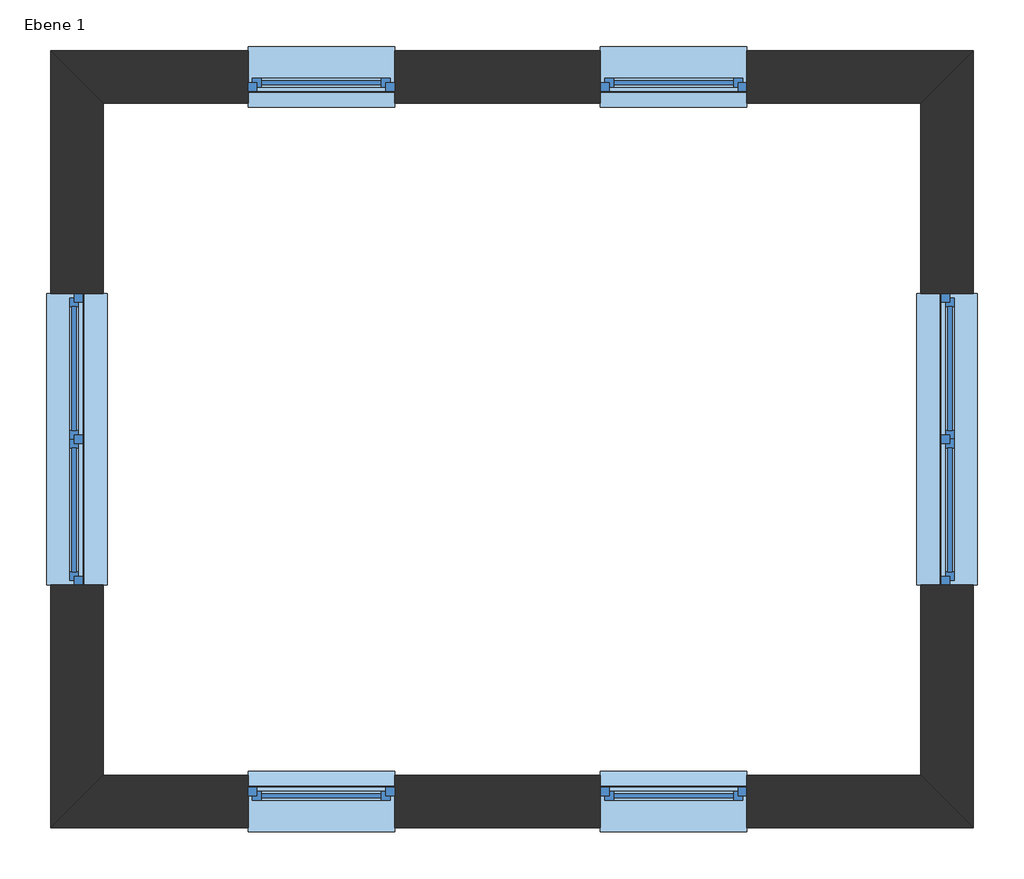
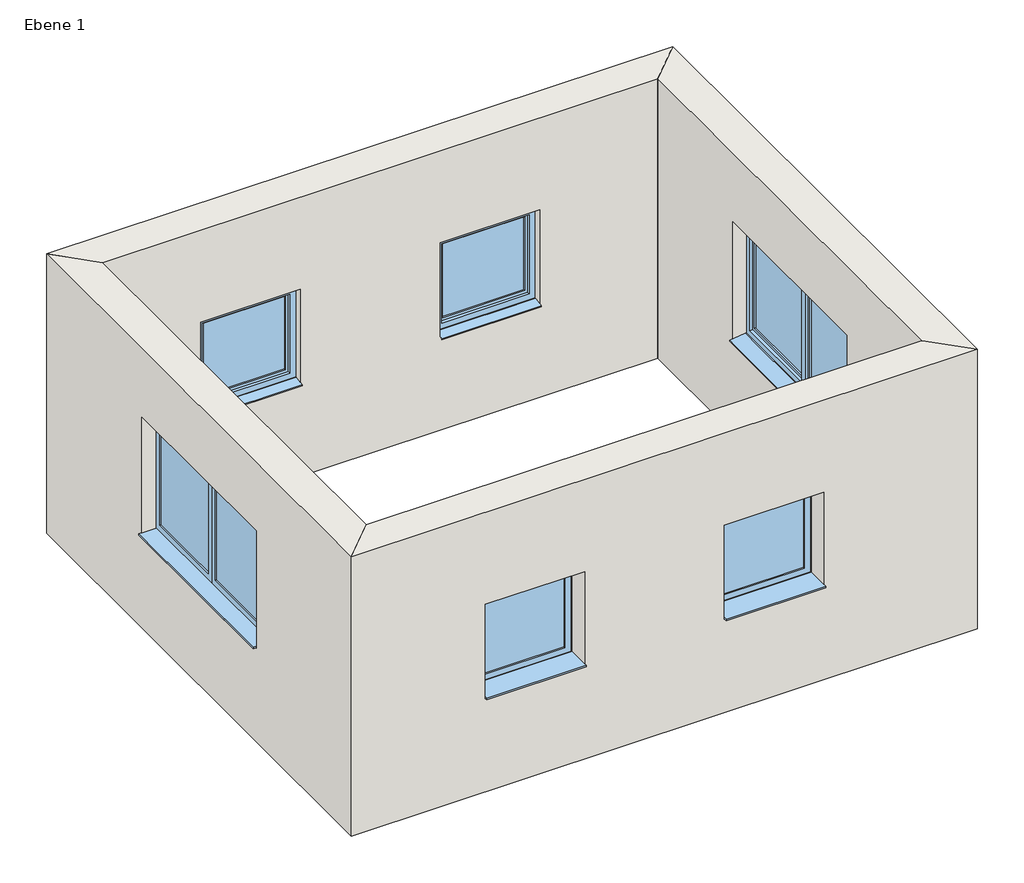
# One storey: 6 windows, 4 walls.
"""IFC4 building model written with IfcOpenShell, lengths in millimetres."""

import ifcopenshell
import ifcopenshell.guid

model = None  # the IFC model being written
_history = None  # IfcOwnerHistory: only IFC2X3 demands one
_inside = {}  # id of a spatial element -> (the spatial element, [elements in it])
_under = {}  # id of a project, library or spatial element -> (it, [spatial elements below it])
_declared = {}  # id of a project -> (the project, [libraries it declares])
_typed = {}  # id of a type object -> (the type object, [elements of that type])
_made_of = {}  # id of a material, layer set ... -> (it, [elements and type objects made of it])


def new_model(schema):
    """Start an empty IFC model of exactly this schema.

    Asked for "IFC4X3", IfcOpenShell would pick the latest addendum, in which some entities
    have other attributes; the version numbers below select the first issue.
    IFC2X3 requires an IfcOwnerHistory on every rooted entity: one is made here for all.
    """
    global model, _history
    if schema == "IFC4X3":
        model = ifcopenshell.file(schema_version=(4, 3, 0, 0))
    else:
        model = ifcopenshell.file(schema=schema)
    _inside.clear()
    _under.clear()
    _declared.clear()
    _typed.clear()
    _made_of.clear()
    _history = None
    if model.schema == "IFC2X3":
        org = make("IfcOrganization", Name="unknown")
        user = make(
            "IfcPersonAndOrganization",
            ThePerson=make("IfcPerson", FamilyName="unknown"),
            TheOrganization=org,
        )
        app = make(
            "IfcApplication",
            ApplicationDeveloper=org,
            Version="unknown",
            ApplicationFullName="unknown",
            ApplicationIdentifier="unknown",
        )
        _history = make(
            "IfcOwnerHistory",
            OwningUser=user,
            OwningApplication=app,
            ChangeAction="ADDED",
            CreationDate=0,
        )
    return model


def make(cls, **values):
    """One entity of the class cls with the attributes given. An attribute that is None is left unset."""
    return model.create_entity(
        cls, **{name: value for name, value in values.items() if value is not None}
    )


def rooted(cls, **values):
    """An entity with a GlobalId (a new one), such as an element, a storey or a relation."""
    return make(cls, GlobalId=ifcopenshell.guid.new(), OwnerHistory=_history, **values)


def si_unit(unit_type, name, prefix=None):
    """IfcSIUnit, for example si_unit("LENGTHUNIT", "METRE", prefix="MILLI")."""
    return make("IfcSIUnit", UnitType=unit_type, Prefix=prefix, Name=name)


def assignment(units):
    """IfcUnitAssignment: the units of a project."""
    return None if units is None else make("IfcUnitAssignment", Units=units)


def point(xyz):
    """IfcCartesianPoint."""
    return None if xyz is None else make("IfcCartesianPoint", Coordinates=xyz)


def direction(xyz):
    """IfcDirection."""
    return None if xyz is None else make("IfcDirection", DirectionRatios=xyz)


def frame(location, z_axis=None, x_axis=None):
    """IfcAxis2Placement3D, a coordinate frame: its origin and axes. An axis left out is left unset."""
    return make(
        "IfcAxis2Placement3D",
        Location=point(location),
        Axis=direction(z_axis),
        RefDirection=direction(x_axis),
    )


def origin():
    """The frame at (0, 0, 0) with its axes left unset."""
    return frame((0.0, 0.0, 0.0))


def place(relative_to, where):
    """IfcLocalPlacement: puts the frame where relative to a parent placement (None: the world)."""
    return make(
        "IfcLocalPlacement", PlacementRelTo=relative_to, RelativePlacement=where
    )


def context(
    kind, dimensions, precision=None, world=None, true_north=None, identifier=None
):
    """IfcGeometricRepresentationContext, for example the 3D "Model" context."""
    return make(
        "IfcGeometricRepresentationContext",
        ContextIdentifier=identifier,
        ContextType=kind,
        CoordinateSpaceDimension=dimensions,
        Precision=precision,
        WorldCoordinateSystem=world,
        TrueNorth=true_north,
    )


def project(units=None, contexts=None):
    """IfcProject with its units and contexts."""
    return rooted(
        "IfcProject",
        Name="project",
        RepresentationContexts=contexts,
        UnitsInContext=assignment(units),
    )


def spatial(cls, under=None, at=None, **own):
    """A site, building, storey or space (cls), placed at a placement, below another one or the project."""
    s = rooted(cls, ObjectPlacement=at, **own)
    if under is not None:
        _under.setdefault(under.id(), (under, []))[1].append(s)
    return s


def polyline(points):
    """IfcPolyline through the points."""
    return make("IfcPolyline", Points=[point(p) for p in points])


def outline(outer, holes=None, kind="AREA"):
    """IfcArbitraryClosedProfileDef: a profile drawn as a closed curve; with holes, ...WithVoids."""
    if holes is None:
        return make("IfcArbitraryClosedProfileDef", ProfileType=kind, OuterCurve=outer)
    return make(
        "IfcArbitraryProfileDefWithVoids",
        ProfileType=kind,
        OuterCurve=outer,
        InnerCurves=holes,
    )


def extrude(swept, where, along, depth):
    """IfcExtrudedAreaSolid: the profile swept, set in the frame where, extruded along a direction by depth."""
    return make(
        "IfcExtrudedAreaSolid",
        SweptArea=swept,
        Position=where,
        ExtrudedDirection=direction(along),
        Depth=depth,
    )


def faces_of(points, faces, orient=None, outer=None):
    """IfcFace entities. A face is a list of loops; a loop is a list of indices into points, from 0.

    orient and outer hold one flag for each loop. By default every Orientation is true, the
    first loop of a face is its IfcFaceOuterBound and the others are IfcFaceBound.
    """
    made = []
    for i, loops in enumerate(faces):
        bounds = []
        for j, loop in enumerate(loops):
            is_outer = j == 0 if outer is None else outer[i][j]
            bounds.append(
                make(
                    "IfcFaceOuterBound" if is_outer else "IfcFaceBound",
                    Bound=make("IfcPolyLoop", Polygon=[points[k] for k in loop]),
                    Orientation=True if orient is None else orient[i][j],
                )
            )
        made.append(make("IfcFace", Bounds=bounds))
    return made


def faceted_brep(points, faces, orient=None, outer=None, voids=None):
    """IfcFacetedBrep: a solid bounded by flat faces; with voids (closed shells), ...WithVoids."""
    shared = [point(p) for p in points]
    hull = make("IfcClosedShell", CfsFaces=faces_of(shared, faces, orient, outer))
    if voids is None:
        return make("IfcFacetedBrep", Outer=hull)
    return make(
        "IfcFacetedBrepWithVoids",
        Outer=hull,
        Voids=[
            make(cls, CfsFaces=faces_of(shared, fs, o, b)) for cls, fs, o, b in voids
        ],
    )


def shape(context_of_items, identifier, shape_type, items):
    """IfcShapeRepresentation: the items that make up one representation, for example the "Body"."""
    return make(
        "IfcShapeRepresentation",
        ContextOfItems=context_of_items,
        RepresentationIdentifier=identifier,
        RepresentationType=shape_type,
        Items=items,
    )


def source(mapping_origin, context_of_items, identifier, shape_type, items):
    """IfcRepresentationMap: a shape defined once, which mapped items show again and again."""
    return make(
        "IfcRepresentationMap",
        MappingOrigin=mapping_origin,
        MappedRepresentation=shape(context_of_items, identifier, shape_type, items),
    )


def transform(
    local_origin,
    x_axis=None,
    y_axis=None,
    z_axis=None,
    scale=None,
    scale2=None,
    scale3=None,
    uniform=True,
):
    """IfcCartesianTransformationOperator3D, or its non-uniform kind. x_axis, y_axis, z_axis: its Axis1, 2, 3."""
    if uniform:
        return make(
            "IfcCartesianTransformationOperator3D",
            Axis1=direction(x_axis),
            Axis2=direction(y_axis),
            LocalOrigin=point(local_origin),
            Scale=scale,
            Axis3=direction(z_axis),
        )
    return make(
        "IfcCartesianTransformationOperator3DnonUniform",
        Axis1=direction(x_axis),
        Axis2=direction(y_axis),
        LocalOrigin=point(local_origin),
        Scale=scale,
        Axis3=direction(z_axis),
        Scale2=scale2,
        Scale3=scale3,
    )


def mapped(mapping_source, mapping_target):
    """IfcMappedItem: shows the shape of a source again, moved by a transform."""
    return make(
        "IfcMappedItem", MappingSource=mapping_source, MappingTarget=mapping_target
    )


def made_of(thing, what):
    """Note that an element or type object is made of a material, layer set ...; save() writes the relation."""
    if what is not None:
        _made_of.setdefault(what.id(), (what, []))[1].append(thing)
    return thing


def element(
    cls,
    number,
    at=None,
    inside=None,
    cuts=None,
    type_object=None,
    material=None,
    context=None,
    identifier="Body",
    shape_type=None,
    held_by="IfcProductDefinitionShape",
    body=None,
    shapes=None,
    **own,
):
    """One element of the class cls, such as IfcWall. Its Tag is "e" and its number.

    at: its placement. inside: the storey or other place that contains it. cuts: it is an
    opening in that element (IfcRelVoidsElement). A single representation is given by context,
    identifier, shape_type and body (its items); several are given by shapes. held_by: the class
    of the entity that holds the representations. save() writes the other relations.
    """
    e = rooted(cls, Tag="e%d" % number, ObjectPlacement=at, **own)
    if body is not None:
        shapes = [shape(context, identifier, shape_type, body)]
    if shapes is not None:
        e.Representation = make(held_by, Representations=shapes)
    if inside is not None:
        _inside.setdefault(inside.id(), (inside, []))[1].append(e)
    if cuts is not None:
        rooted(
            "IfcRelVoidsElement", RelatingBuildingElement=cuts, RelatedOpeningElement=e
        )
    if type_object is not None:
        _typed.setdefault(type_object.id(), (type_object, []))[1].append(e)
    return made_of(e, material)


def aggregate(whole, parts):
    """IfcRelAggregates: a whole, such as a stair, and the parts it consists of."""
    return rooted("IfcRelAggregates", RelatingObject=whole, RelatedObjects=parts)


def save(model, path):
    """Write the relations noted so far, then the file.

    IfcRelAggregates (storeys below a building ...), IfcRelContainedInSpatialStructure (elements
    in a storey), IfcRelDefinesByType, IfcRelAssociatesMaterial and IfcRelDeclares: one each for
    every whole, place, type object, material and project.
    """
    for whole, parts in _under.values():
        aggregate(whole, parts)
    for where, things in _inside.values():
        rooted(
            "IfcRelContainedInSpatialStructure",
            RelatedElements=things,
            RelatingStructure=where,
        )
    for kind, things in _typed.values():
        rooted("IfcRelDefinesByType", RelatedObjects=things, RelatingType=kind)
    for what, things in _made_of.values():
        rooted("IfcRelAssociatesMaterial", RelatedObjects=things, RelatingMaterial=what)
    for by, libraries in _declared.values():
        rooted("IfcRelDeclares", RelatingContext=by, RelatedDefinitions=libraries)
    model.write(path)


def fenster_1_flg_variabel_fenster_1_flg_variabel_3_8a378bad(model_context):
    return source(origin(), model_context, "Body", "SolidModel", [
        extrude(outline(polyline([(2010.0, 505.0), (2010.0, -505.0), (1000.0, -505.0), (1000.0, 505.0), (2010.0, 505.0)]), holes=[polyline([(1930.0, 445.0), (1080.0, 445.0), (1080.0, -445.0), (1930.0, -445.0), (1930.0, 445.0)])]), frame((0.0, 40.0, 0.0), z_axis=(0.0, 1.0, 0.0), x_axis=(0.0, 0.0, 1.0)), (0.0, 0.0, 1.0), 60.0),
        faceted_brep([(475.0, 40.0, 1960.0), (475.0, 10.0, 1960.0), (475.0, 10.0, 1050.0), (475.0, 40.0, 1050.0), (-475.0, 10.0, 1960.0), (-475.0, 10.0, 1050.0), (415.0, 10.0, 1110.0), (-415.0, 10.0, 1110.0), (-415.0, 10.0, 1900.0), (415.0, 10.0, 1900.0), (-475.0, 40.0, 1050.0), (-475.0, 40.0, 1960.0), (445.0, 40.0, 1930.0), (-445.0, 40.0, 1930.0), (-445.0, 40.0, 1080.0), (445.0, 40.0, 1080.0), (445.0, 70.0, 1930.0), (445.0, 70.0, 1080.0), (-445.0, 70.0, 1080.0), (-445.0, 70.0, 1930.0), (415.0, 70.0, 1900.0), (-415.0, 70.0, 1900.0), (-415.0, 70.0, 1110.0), (415.0, 70.0, 1110.0)], [[[0, 1, 2, 3]], [[1, 4, 5, 2], [6, 7, 8, 9]], [[3, 2, 5, 10]], [[3, 10, 11, 0], [12, 13, 14, 15]], [[16, 12, 15, 17]], [[17, 15, 14, 18]], [[17, 18, 19, 16], [20, 21, 22, 23]], [[9, 20, 23, 6]], [[6, 23, 22, 7]], [[10, 5, 4, 11]], [[18, 14, 13, 19]], [[7, 22, 21, 8]], [[11, 4, 1, 0]], [[19, 13, 12, 16]], [[8, 21, 20, 9]]]),
        extrude(outline(polyline([(-505.0, -210.0), (-505.0, 40.0), (505.0, 40.0), (505.0, -210.0), (-505.0, -210.0)])), frame((0.0, 0.0, 1005.0), z_axis=(0.0, 0.0, 1.0), x_axis=(1.0, 0.0, 0.0)), (0.0, 0.0, 1.0), 15.0),
        extrude(outline(polyline([(110.0221543, 1020.0), (210.0, 1000.0), (210.0, 990.0), (208.0, 990.0), (208.0, 998.3604634), (109.8240723, 1018.0), (100.0, 1018.0), (100.0, 1020.0), (110.0221543, 1020.0)])), frame((-505.0, 0.0, 0.0), z_axis=(1.0, 0.0, 0.0), x_axis=(0.0, 1.0, 0.0)), (0.0, 0.0, 1.0), 1010.0),
        extrude(outline(polyline([(415.0, 25.0), (-415.0, 25.0), (-415.0, 55.0), (415.0, 55.0), (415.0, 25.0)])), frame((0.0, 0.0, 1110.0), z_axis=(0.0, 0.0, 1.0), x_axis=(1.0, 0.0, 0.0)), (0.0, 0.0, 1.0), 790.0),
    ])


def fenster_2_flg_variabel_fenster_2_flg_variabel_3_03287464(model_context):
    return source(origin(), model_context, "Body", "SolidModel", [
        extrude(outline(polyline([(60.0, -5.0), (915.0, -5.0), (915.0, -35.0), (60.0, -35.0), (60.0, -5.0)])), frame((0.0, 0.0, 1110.0), z_axis=(0.0, 0.0, 1.0), x_axis=(1.0, 0.0, 0.0)), (0.0, 0.0, 1.0), 1040.0),
        extrude(outline(polyline([(-915.0, -5.0), (-60.0, -5.0), (-60.0, -35.0), (-915.0, -35.0), (-915.0, -5.0)])), frame((0.0, 0.0, 1110.0), z_axis=(0.0, 0.0, 1.0), x_axis=(1.0, 0.0, 0.0)), (0.0, 0.0, 1.0), 1040.0),
        extrude(outline(polyline([(-1005.0, -210.0), (-1005.0, -20.0), (1005.0, -20.0), (1005.0, -210.0), (-1005.0, -210.0)])), frame((0.0, 0.0, 1005.0), z_axis=(0.0, 0.0, 1.0), x_axis=(1.0, 0.0, 0.0)), (0.0, 0.0, 1.0), 15.0),
        extrude(outline(polyline([(50.0221543, 1020.0), (210.0, 1000.0), (210.0, 990.0), (208.0, 990.0), (208.0, 998.3604634), (49.8240723, 1018.0), (40.0, 1018.0), (40.0, 1020.0), (50.0221543, 1020.0)])), frame((-1005.0, 0.0, 0.0), z_axis=(1.0, 0.0, 0.0), x_axis=(0.0, 1.0, 0.0)), (0.0, 0.0, 1.0), 2010.0),
        extrude(outline(polyline([(30.0, -20.0), (-30.0, -20.0), (-30.0, 40.0), (30.0, 40.0), (30.0, -20.0)])), frame((0.0, 0.0, 1080.0), z_axis=(0.0, 0.0, 1.0), x_axis=(1.0, 0.0, 0.0)), (0.0, 0.0, 1.0), 1100.0),
        extrude(outline(polyline([(2260.0, -1005.0), (1000.0, -1005.0), (1000.0, 1005.0), (2260.0, 1005.0), (2260.0, -1005.0)]), holes=[polyline([(2180.0, -945.0), (2180.0, 945.0), (1080.0, 945.0), (1080.0, -945.0), (2180.0, -945.0)])]), frame((0.0, -20.0, 0.0), z_axis=(0.0, 1.0, 0.0), x_axis=(0.0, 0.0, 1.0)), (0.0, 0.0, 1.0), 60.0),
        faceted_brep([(-945.0, -20.0, 1080.0), (-945.0, 10.0, 1080.0), (-30.0, 10.0, 1080.0), (-30.0, -20.0, 1080.0), (-30.0, 10.0, 2180.0), (-30.0, -20.0, 2180.0), (-945.0, 10.0, 2180.0), (-60.0, 10.0, 2150.0), (-915.0, 10.0, 2150.0), (-915.0, 10.0, 1110.0), (-60.0, 10.0, 1110.0), (0.0, -20.0, 1050.0), (-975.0, -20.0, 1050.0), (-975.0, -20.0, 2210.0), (0.0, -20.0, 2210.0), (-945.0, -20.0, 2180.0), (-975.0, -50.0, 1050.0), (0.0, -50.0, 1050.0), (0.0, -50.0, 2210.0), (-975.0, -50.0, 2210.0), (-60.0, -50.0, 1110.0), (-915.0, -50.0, 1110.0), (-915.0, -50.0, 2150.0), (-60.0, -50.0, 2150.0)], [[[0, 1, 2, 3]], [[3, 2, 4, 5]], [[2, 1, 6, 4], [7, 8, 9, 10]], [[11, 12, 13, 14], [5, 15, 0, 3]], [[16, 12, 11, 17]], [[17, 11, 14, 18]], [[18, 19, 16, 17], [20, 21, 22, 23]], [[9, 21, 20, 10]], [[10, 20, 23, 7]], [[15, 6, 1, 0]], [[19, 13, 12, 16]], [[8, 22, 21, 9]], [[5, 4, 6, 15]], [[18, 14, 13, 19]], [[7, 23, 22, 8]]]),
        faceted_brep([(30.0, -20.0, 1080.0), (30.0, 10.0, 1080.0), (945.0, 10.0, 1080.0), (945.0, -20.0, 1080.0), (945.0, 10.0, 2180.0), (945.0, -20.0, 2180.0), (30.0, 10.0, 2180.0), (915.0, 10.0, 2150.0), (60.0, 10.0, 2150.0), (60.0, 10.0, 1110.0), (915.0, 10.0, 1110.0), (975.0, -20.0, 1050.0), (0.0, -20.0, 1050.0), (0.0, -20.0, 2210.0), (975.0, -20.0, 2210.0), (30.0, -20.0, 2180.0), (0.0, -50.0, 1050.0), (975.0, -50.0, 1050.0), (975.0, -50.0, 2210.0), (0.0, -50.0, 2210.0), (915.0, -50.0, 1110.0), (60.0, -50.0, 1110.0), (60.0, -50.0, 2150.0), (915.0, -50.0, 2150.0)], [[[0, 1, 2, 3]], [[3, 2, 4, 5]], [[2, 1, 6, 4], [7, 8, 9, 10]], [[11, 12, 13, 14], [5, 15, 0, 3]], [[16, 12, 11, 17]], [[17, 11, 14, 18]], [[18, 19, 16, 17], [20, 21, 22, 23]], [[9, 21, 20, 10]], [[10, 20, 23, 7]], [[15, 6, 1, 0]], [[19, 13, 12, 16]], [[8, 22, 21, 9]], [[5, 4, 6, 15]], [[18, 14, 13, 19]], [[7, 23, 22, 8]]]),
    ])


model = new_model("IFC4")

# Units and contexts
model_context = context("Model", 3, world=origin())
ifc_project = project(units=[si_unit("LENGTHUNIT", "METRE", prefix="MILLI")], contexts=[model_context])

# Site, building, storey
site = spatial("IfcSite", under=ifc_project)
building = spatial("IfcBuilding", under=site)
storey = spatial("IfcBuildingStorey", under=building, Name="Ebene 1", Elevation=3000.0)

# Walls
placement = place(None, origin())
element("IfcWall", 1, ObjectType="MW 24.0 WD 12.0", at=placement, inside=storey, context=model_context, shape_type="Brep", body=[
    faceted_brep([(-3766.4979049, 4044.3692517, 3000.0), (1873.5020951, 4044.3692517, 3000.0), (1873.5020951, 4044.3692517, 6000.0), (-3766.4979049, 4044.3692517, 6000.0), (673.5020951, 4044.3692517, 4000.0), (-336.4979049, 4044.3692517, 4000.0), (-336.4979049, 4044.3692517, 5010.0), (673.5020951, 4044.3692517, 5010.0), (-1756.4979049, 4044.3692517, 4000.0), (-2766.4979049, 4044.3692517, 4000.0), (-2766.4979049, 4044.3692517, 5010.0), (-1756.4979049, 4044.3692517, 5010.0), (-4126.4979049, 4404.3692517, 3000.0), (-4126.4979049, 4404.3692517, 6000.0), (2233.5020951, 4404.3692517, 6000.0), (2233.5020951, 4404.3692517, 3000.0), (673.5020951, 4404.3692517, 4000.0), (673.5020951, 4404.3692517, 5010.0), (-336.4979049, 4404.3692517, 5010.0), (-336.4979049, 4404.3692517, 4000.0), (-1756.4979049, 4404.3692517, 4000.0), (-1756.4979049, 4404.3692517, 5010.0), (-2766.4979049, 4404.3692517, 5010.0), (-2766.4979049, 4404.3692517, 4000.0)], [[[0, 1, 2, 3], [4, 5, 6, 7], [8, 9, 10, 11]], [[12, 13, 14, 15], [16, 17, 18, 19], [20, 21, 22, 23]], [[1, 0, 12, 15]], [[3, 2, 14, 13]], [[2, 1, 15, 14]], [[0, 3, 13, 12]], [[17, 16, 4, 7]], [[18, 17, 7, 6]], [[19, 18, 6, 5]], [[16, 19, 5, 4]], [[21, 20, 8, 11]], [[22, 21, 11, 10]], [[23, 22, 10, 9]], [[20, 23, 9, 8]]]),
])
element("IfcWall", 2, ObjectType="MW 24.0 WD 12.0", at=placement, inside=storey, context=model_context, shape_type="Brep", body=[
    faceted_brep([(1873.5020951, 4044.3692517, 3000.0), (1873.5020951, -595.6307483, 3000.0), (1873.5020951, -595.6307483, 6000.0), (1873.5020951, 4044.3692517, 6000.0), (1873.5020951, 719.3692517, 4000.0), (1873.5020951, 2729.3692517, 4000.0), (1873.5020951, 2729.3692517, 5260.0), (1873.5020951, 719.3692517, 5260.0), (2233.5020951, 4404.3692517, 3000.0), (2233.5020951, 4404.3692517, 6000.0), (2233.5020951, -955.6307483, 6000.0), (2233.5020951, -955.6307483, 3000.0), (2233.5020951, 719.3692517, 4000.0), (2233.5020951, 719.3692517, 5260.0), (2233.5020951, 2729.3692517, 5260.0), (2233.5020951, 2729.3692517, 4000.0)], [[[0, 1, 2, 3], [4, 5, 6, 7]], [[8, 9, 10, 11], [12, 13, 14, 15]], [[1, 0, 8, 11]], [[3, 2, 10, 9]], [[0, 3, 9, 8]], [[2, 1, 11, 10]], [[13, 12, 4, 7]], [[14, 13, 7, 6]], [[15, 14, 6, 5]], [[12, 15, 5, 4]]]),
])
element("IfcWall", 3, ObjectType="MW 24.0 WD 12.0", at=placement, inside=storey, context=model_context, shape_type="Brep", body=[
    faceted_brep([(1873.5020951, -595.6307483, 3000.0), (-3766.4979049, -595.6307483, 3000.0), (-3766.4979049, -595.6307483, 6000.0), (1873.5020951, -595.6307483, 6000.0), (-336.4979049, -595.6307483, 4000.0), (673.5020951, -595.6307483, 4000.0), (673.5020951, -595.6307483, 5010.0), (-336.4979049, -595.6307483, 5010.0), (-2766.4979049, -595.6307483, 4000.0), (-1756.4979049, -595.6307483, 4000.0), (-1756.4979049, -595.6307483, 5010.0), (-2766.4979049, -595.6307483, 5010.0), (2233.5020951, -955.6307483, 3000.0), (2233.5020951, -955.6307483, 6000.0), (-4126.4979049, -955.6307483, 6000.0), (-4126.4979049, -955.6307483, 3000.0), (-336.4979049, -955.6307483, 4000.0), (-336.4979049, -955.6307483, 5010.0), (673.5020951, -955.6307483, 5010.0), (673.5020951, -955.6307483, 4000.0), (-2766.4979049, -955.6307483, 4000.0), (-2766.4979049, -955.6307483, 5010.0), (-1756.4979049, -955.6307483, 5010.0), (-1756.4979049, -955.6307483, 4000.0)], [[[0, 1, 2, 3], [4, 5, 6, 7], [8, 9, 10, 11]], [[12, 13, 14, 15], [16, 17, 18, 19], [20, 21, 22, 23]], [[1, 0, 12, 15]], [[3, 2, 14, 13]], [[0, 3, 13, 12]], [[2, 1, 15, 14]], [[17, 16, 4, 7]], [[18, 17, 7, 6]], [[19, 18, 6, 5]], [[16, 19, 5, 4]], [[21, 20, 8, 11]], [[22, 21, 11, 10]], [[23, 22, 10, 9]], [[20, 23, 9, 8]]]),
])
element("IfcWall", 4, ObjectType="MW 24.0 WD 12.0", at=placement, inside=storey, context=model_context, shape_type="Brep", body=[
    faceted_brep([(-3766.4979049, -595.6307483, 3000.0), (-3766.4979049, 4044.3692517, 3000.0), (-3766.4979049, 4044.3692517, 6000.0), (-3766.4979049, -595.6307483, 6000.0), (-3766.4979049, 2729.3692517, 4000.0), (-3766.4979049, 719.3692517, 4000.0), (-3766.4979049, 719.3692517, 5260.0), (-3766.4979049, 2729.3692517, 5260.0), (-4126.4979049, -955.6307483, 3000.0), (-4126.4979049, -955.6307483, 6000.0), (-4126.4979049, 4404.3692517, 6000.0), (-4126.4979049, 4404.3692517, 3000.0), (-4126.4979049, 2729.3692517, 4000.0), (-4126.4979049, 2729.3692517, 5260.0), (-4126.4979049, 719.3692517, 5260.0), (-4126.4979049, 719.3692517, 4000.0)], [[[0, 1, 2, 3], [4, 5, 6, 7]], [[8, 9, 10, 11], [12, 13, 14, 15]], [[1, 0, 8, 11]], [[3, 2, 10, 9]], [[2, 1, 11, 10]], [[0, 3, 9, 8]], [[13, 12, 4, 7]], [[14, 13, 7, 6]], [[15, 14, 6, 5]], [[12, 15, 5, 4]]]),
])

# Windows
fenster_1_flg_variabel_fenster_1_flg_variabel_3_shape = fenster_1_flg_variabel_fenster_1_flg_variabel_3_8a378bad(model_context)
element("IfcWindow", 5, ObjectType="Fenster 1-flg - Variabel : Fenster 1-flg - Variabel 3", at=placement, inside=storey, context=model_context, shape_type="MappedRepresentation", body=[
    mapped(fenster_1_flg_variabel_fenster_1_flg_variabel_3_shape, transform((168.5020951, -775.6307483, 3000.0), x_axis=(1.0, 0.0, 0.0), y_axis=(0.0, 1.0, 0.0), z_axis=(0.0, 0.0, 1.0))),
])
element("IfcWindow", 6, ObjectType="Fenster 1-flg - Variabel : Fenster 1-flg - Variabel 3", at=placement, inside=storey, context=model_context, shape_type="MappedRepresentation", body=[
    mapped(fenster_1_flg_variabel_fenster_1_flg_variabel_3_shape, transform((-2261.4979049, -775.6307483, 3000.0), x_axis=(1.0, 0.0, 0.0), y_axis=(0.0, 1.0, 0.0), z_axis=(0.0, 0.0, 1.0))),
])
element("IfcWindow", 7, ObjectType="Fenster 1-flg - Variabel : Fenster 1-flg - Variabel 3", at=placement, inside=storey, context=model_context, shape_type="MappedRepresentation", body=[
    mapped(fenster_1_flg_variabel_fenster_1_flg_variabel_3_shape, transform((168.5020951, 4224.3692517, 3000.0), x_axis=(-1.0, 0.0, 0.0), y_axis=(0.0, -1.0, 0.0), z_axis=(0.0, 0.0, 1.0))),
])
element("IfcWindow", 8, ObjectType="Fenster 1-flg - Variabel : Fenster 1-flg - Variabel 3", at=placement, inside=storey, context=model_context, shape_type="MappedRepresentation", body=[
    mapped(fenster_1_flg_variabel_fenster_1_flg_variabel_3_shape, transform((-2261.4979049, 4224.3692517, 3000.0), x_axis=(-1.0, 0.0, 0.0), y_axis=(0.0, -1.0, 0.0), z_axis=(0.0, 0.0, 1.0))),
])
fenster_2_flg_variabel_fenster_2_flg_variabel_3_shape = fenster_2_flg_variabel_fenster_2_flg_variabel_3_03287464(model_context)
element("IfcWindow", 9, ObjectType="Fenster 2-flg - Variabel : Fenster 2-flg - Variabel 3", at=placement, inside=storey, context=model_context, shape_type="MappedRepresentation", body=[
    mapped(fenster_2_flg_variabel_fenster_2_flg_variabel_3_shape, transform((2053.5020951, 1724.3692517, 3000.0), x_axis=(0.0, 1.0, 0.0), y_axis=(-1.0, 0.0, 0.0), z_axis=(0.0, 0.0, 1.0))),
])
element("IfcWindow", 10, ObjectType="Fenster 2-flg - Variabel : Fenster 2-flg - Variabel 3", at=placement, inside=storey, context=model_context, shape_type="MappedRepresentation", body=[
    mapped(fenster_2_flg_variabel_fenster_2_flg_variabel_3_shape, transform((-3946.4979049, 1724.3692517, 3000.0), x_axis=(0.0, -1.0, 0.0), y_axis=(1.0, 0.0, 0.0), z_axis=(0.0, 0.0, 1.0))),
])

save(model, "model.ifc")

# Revit data of these elements
# Type "MW 24.0 WD 12.0"
#   Type Comments = "Mehrschaliges Mauerwerk"
#   Description = "Mauerwerk 24.0 cm, Wärmedämmung 12.0 cm"
#   Layers, outside or top first: 0.120 m "Wärmedämmung - hart" (function 3); 0.240 m "Mauerwerk - Ziegel, verputzt" (function 1)
# Type "Fenster 1-flg - Variabel : Fenster 1-flg - Variabel 3"
#   Type Mark = "52"
#   Operation = "SinglePanel"
#   Construction Type Id = "GSP4R"
#   Keynote = "16.05.01"
#   Analytic Construction = "1/8 Zoll Pilkington-Verglasung einfach"
#   Cost = 78.2
#   Visual Light Transmittance = 0.9
#   Höhe oberer  Rahmen = 0.080 m
#   Solar Heat Gain Coefficient = 0.86
#   Tiefe Flügel = 0.060 m
#   Rough Width [instance default] = 1.010 m
#   Rough Height [instance default] = 1.010 m
#   Rahmenhöhe unten = 0.080 m
#   Heat Transfer Coefficient (U) = 6.7069 W/(m²·K)
#   Rahmentiefe = 0.060 m
#   Rahmenbreite = 0.060 m
#   Height [instance default] = 1.010 m
#   Flügelbreite = 0.060 m
#   Einbautiefe (von außen) [instance default] = 0.080 m
#   Width [instance default] = 1.010 m
#   Define Thermal Properties by = 1
#   Öffnungsrichtung oben [instance default] = yes
#   Öffnungsrichtung in Draufsicht anzeigen [instance default] = no
#   Klappflügel [instance default] = no
#   Drehflügel 1 [instance default] = yes
#   Fensterflügel [instance default] = none
#   Innere Fensterbank [instance default] = none
#   Glas [instance default] = none
#   Bild [instance default] = none
#   Äußere Fensterbank [instance default] = none
#   Wall Closure = (empty or 0)
# Type "Fenster 2-flg - Variabel : Fenster 2-flg - Variabel 3"
#   Type Mark = "53"
#   Operation = "DoublePanelVertical"
#   Construction Type Id = "GSP4R"
#   Keynote = "16.05.01"
#   Analytic Construction = "1/8 Zoll Pilkington-Verglasung einfach"
#   Cost = 130.98
#   Visual Light Transmittance = 0.9
#   Solar Heat Gain Coefficient = 0.78
#   Rough Width [instance default] = 2.010 m
#   Rough Height [instance default] = 1.260 m
#   Heat Transfer Coefficient (U) = 3.6886 W/(m²·K)
#   Rahmentiefe = 0.060 m
#   Rahmenhöhe unten = 0.080 m
#   Höhe oberer  Rahmen = 0.080 m
#   Rahmenbreite = 0.060 m
#   Height [instance default] = 1.260 m
#   Tiefe Flügel = 0.060 m
#   Flügelbreite = 0.060 m
#   Einbautiefe (von außen) [instance default] = 0.140 m
#   Width [instance default] = 2.010 m
#   Define Thermal Properties by = 1
#   Öffnungsrichtung oben [instance default] = yes
#   Öffnungsrichtung in Draufsicht anzeigen [instance default] = no
#   Drehflügel 1 [instance default] = yes
#   Bild [instance default] = none
#   Glas [instance default] = none
#   Fensterflügel [instance default] = none
#   Äußere Fensterbank [instance default] = none
#   Innere Fensterbank [instance default] = none
#   Wall Closure = (empty or 0)
# Elements 1, 2, 3, 4 (IfcWall, "MW 24.0 WD 12.0")
#   Comments = ""
#   Top Offset = 0.000 m
#   Base Offset = 0.000 m
#   Unconnected Height = 3.000 m
#   wall height = 3.000 m
#   Phase Created = Phase 1
#   Base Constraint = Ebene 1
#   Materials on its faces: "Vorgabe - Wand", "Mauerwerk - Ziegel, verputzt", "Wärmedämmung - hart"
# Element 5 (IfcWindow, "Fenster 1-flg - Variabel : Fenster 1-flg - Variabel 3")
#   Mark = "2"
#   Rough Height = 1.010 m
#   Rough Width = 1.010 m
#   Height = 1.010 m
#   Einbautiefe (von außen) = 0.080 m
#   Width = 1.010 m
#   Öffnungsrichtung oben = yes
#   Öffnungsrichtung in Draufsicht anzeigen = no
#   Klappflügel = no
#   Drehflügel 1 = yes
#   Äußere Fensterbank = none
#   Innere Fensterbank = none
#   Glas = none
#   Fensterflügel = none
#   Bild = none
#   Phase Created = Phase 1
#   Materials on its faces: "Kunststoff - Weiß", "Holz - Birke", "Glas"
# Element 6 (IfcWindow, "Fenster 1-flg - Variabel : Fenster 1-flg - Variabel 3")
#   Mark = "3"
#   Rough Height = 1.010 m
#   Rough Width = 1.010 m
#   Height = 1.010 m
#   Einbautiefe (von außen) = 0.080 m
#   Width = 1.010 m
#   Öffnungsrichtung oben = yes
#   Öffnungsrichtung in Draufsicht anzeigen = no
#   Klappflügel = no
#   Drehflügel 1 = yes
#   Äußere Fensterbank = none
#   Innere Fensterbank = none
#   Glas = none
#   Fensterflügel = none
#   Bild = none
#   Phase Created = Phase 1
#   Materials on its faces: "Kunststoff - Weiß", "Holz - Birke", "Glas"
# Element 7 (IfcWindow, "Fenster 1-flg - Variabel : Fenster 1-flg - Variabel 3")
#   Mark = "4"
#   Rough Height = 1.010 m
#   Rough Width = 1.010 m
#   Height = 1.010 m
#   Einbautiefe (von außen) = 0.080 m
#   Width = 1.010 m
#   Öffnungsrichtung oben = yes
#   Öffnungsrichtung in Draufsicht anzeigen = no
#   Klappflügel = no
#   Drehflügel 1 = yes
#   Äußere Fensterbank = none
#   Innere Fensterbank = none
#   Glas = none
#   Fensterflügel = none
#   Bild = none
#   Phase Created = Phase 1
#   Materials on its faces: "Kunststoff - Weiß", "Holz - Birke", "Glas"
# Element 8 (IfcWindow, "Fenster 1-flg - Variabel : Fenster 1-flg - Variabel 3")
#   Mark = "5"
#   Rough Height = 1.010 m
#   Rough Width = 1.010 m
#   Height = 1.010 m
#   Einbautiefe (von außen) = 0.080 m
#   Width = 1.010 m
#   Öffnungsrichtung oben = yes
#   Öffnungsrichtung in Draufsicht anzeigen = no
#   Klappflügel = no
#   Drehflügel 1 = yes
#   Äußere Fensterbank = none
#   Innere Fensterbank = none
#   Glas = none
#   Fensterflügel = none
#   Bild = none
#   Phase Created = Phase 1
#   Materials on its faces: "Kunststoff - Weiß", "Holz - Birke", "Glas"
# Element 9 (IfcWindow, "Fenster 2-flg - Variabel : Fenster 2-flg - Variabel 3")
#   Mark = "8"
#   Rough Height = 1.260 m
#   Rough Width = 2.010 m
#   Height = 1.260 m
#   Einbautiefe (von außen) = 0.140 m
#   Width = 2.010 m
#   Öffnungsrichtung oben = yes
#   Öffnungsrichtung in Draufsicht anzeigen = no
#   Drehflügel 1 = yes
#   Äußere Fensterbank = none
#   Innere Fensterbank = none
#   Glas = none
#   Fensterflügel = none
#   Bild = none
#   Phase Created = Phase 1
#   Materials on its faces: "Kunststoff - Weiß", "Glas", "Holz - Birke"
# Element 10 (IfcWindow, "Fenster 2-flg - Variabel : Fenster 2-flg - Variabel 3")
#   Mark = "9"
#   Rough Height = 1.260 m
#   Rough Width = 2.010 m
#   Height = 1.260 m
#   Einbautiefe (von außen) = 0.140 m
#   Width = 2.010 m
#   Öffnungsrichtung oben = yes
#   Öffnungsrichtung in Draufsicht anzeigen = no
#   Drehflügel 1 = yes
#   Äußere Fensterbank = none
#   Innere Fensterbank = none
#   Glas = none
#   Fensterflügel = none
#   Bild = none
#   Phase Created = Phase 1
#   Materials on its faces: "Kunststoff - Weiß", "Glas", "Holz - Birke"
# Materials
#   "Wärmedämmung - hart": class "Stuck", colour RGB 255 255 255, transparency 0, Description = "Äußere Oberfläche", Cost = 0
#   "Mauerwerk - Ziegel, verputzt": class "Stuck", colour RGB 247 247 247, transparency 0, Cost = 0
#   "Vorgabe - Wand": class "Stuck", colour RGB 128 128 128, transparency 0, Description = "Äußere Oberfläche", Cost = 0
#   "Kunststoff - Weiß": class "Kunststoff", colour RGB 249 249 249, transparency 0, Cost = 0
#   "Holz - Birke": class "Holz", colour RGB 213 164 103, transparency 0, Cost = 0
#   "Glas": class "Glas", colour RGB 0 0 255, transparency 0.75, Comments = "Render-Darstellung nicht aktualisiert ", Cost = 0
